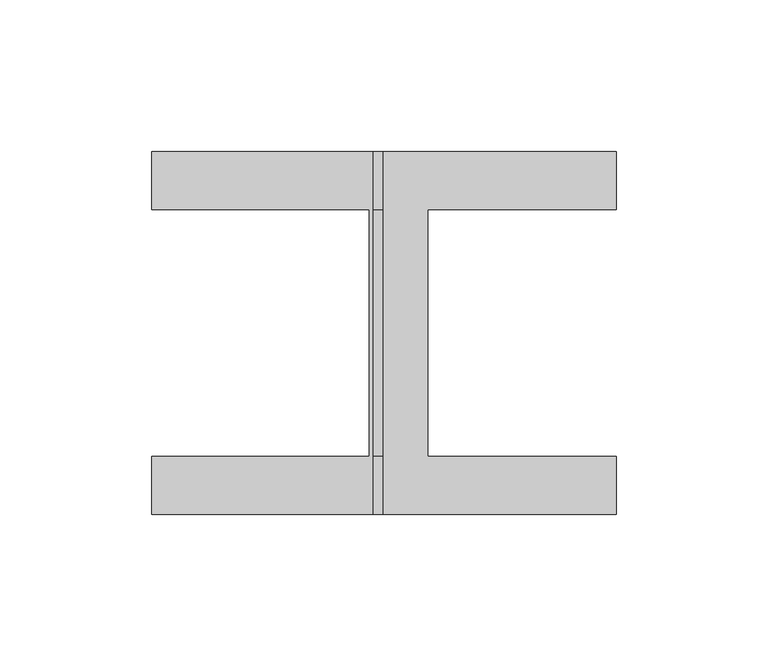
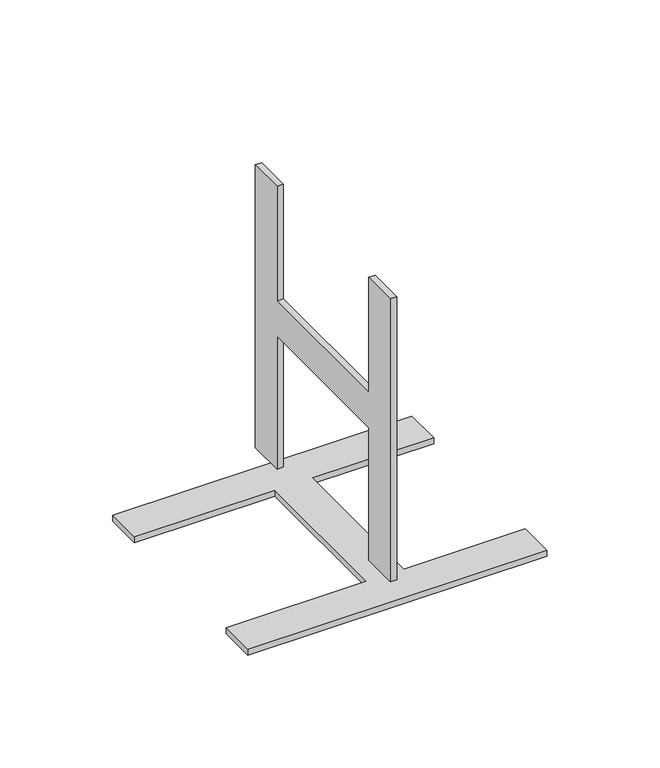
"""IFC4 building model written with IfcOpenShell, lengths in millimetres: proxy geometry, Grid Number2_FedEx : Grid Number2_FedEx."""

import ifcopenshell
import ifcopenshell.guid

model = None  # the IFC model being written
_history = None  # IfcOwnerHistory: only IFC2X3 demands one
_inside = {}  # id of a spatial element -> (the spatial element, [elements in it])
_under = {}  # id of a project, library or spatial element -> (it, [spatial elements below it])
_declared = {}  # id of a project -> (the project, [libraries it declares])
_typed = {}  # id of a type object -> (the type object, [elements of that type])
_made_of = {}  # id of a material, layer set ... -> (it, [elements and type objects made of it])


def new_model(schema):
    """Start an empty IFC model of exactly this schema.

    Asked for "IFC4X3", IfcOpenShell would pick the latest addendum, in which some entities
    have other attributes; the version numbers below select the first issue.
    IFC2X3 requires an IfcOwnerHistory on every rooted entity: one is made here for all.
    """
    global model, _history
    if schema == "IFC4X3":
        model = ifcopenshell.file(schema_version=(4, 3, 0, 0))
    else:
        model = ifcopenshell.file(schema=schema)
    _inside.clear()
    _under.clear()
    _declared.clear()
    _typed.clear()
    _made_of.clear()
    _history = None
    if model.schema == "IFC2X3":
        org = make("IfcOrganization", Name="unknown")
        user = make(
            "IfcPersonAndOrganization",
            ThePerson=make("IfcPerson", FamilyName="unknown"),
            TheOrganization=org,
        )
        app = make(
            "IfcApplication",
            ApplicationDeveloper=org,
            Version="unknown",
            ApplicationFullName="unknown",
            ApplicationIdentifier="unknown",
        )
        _history = make(
            "IfcOwnerHistory",
            OwningUser=user,
            OwningApplication=app,
            ChangeAction="ADDED",
            CreationDate=0,
        )
    return model


def make(cls, **values):
    """One entity of the class cls with the attributes given. An attribute that is None is left unset."""
    return model.create_entity(
        cls, **{name: value for name, value in values.items() if value is not None}
    )


def rooted(cls, **values):
    """An entity with a GlobalId (a new one), such as an element, a storey or a relation."""
    return make(cls, GlobalId=ifcopenshell.guid.new(), OwnerHistory=_history, **values)


def si_unit(unit_type, name, prefix=None):
    """IfcSIUnit, for example si_unit("LENGTHUNIT", "METRE", prefix="MILLI")."""
    return make("IfcSIUnit", UnitType=unit_type, Prefix=prefix, Name=name)


def assignment(units):
    """IfcUnitAssignment: the units of a project."""
    return None if units is None else make("IfcUnitAssignment", Units=units)


def point(xyz):
    """IfcCartesianPoint."""
    return None if xyz is None else make("IfcCartesianPoint", Coordinates=xyz)


def direction(xyz):
    """IfcDirection."""
    return None if xyz is None else make("IfcDirection", DirectionRatios=xyz)


def frame(location, z_axis=None, x_axis=None):
    """IfcAxis2Placement3D, a coordinate frame: its origin and axes. An axis left out is left unset."""
    return make(
        "IfcAxis2Placement3D",
        Location=point(location),
        Axis=direction(z_axis),
        RefDirection=direction(x_axis),
    )


def origin():
    """The frame at (0, 0, 0) with its axes left unset."""
    return frame((0.0, 0.0, 0.0))


def origin_with_axes():
    """The frame at (0, 0, 0) with the z axis (0, 0, 1) and the x axis (1, 0, 0) written out."""
    return frame((0.0, 0.0, 0.0), z_axis=(0.0, 0.0, 1.0), x_axis=(1.0, 0.0, 0.0))


def place(relative_to, where):
    """IfcLocalPlacement: puts the frame where relative to a parent placement (None: the world)."""
    return make(
        "IfcLocalPlacement", PlacementRelTo=relative_to, RelativePlacement=where
    )


def context(
    kind, dimensions, precision=None, world=None, true_north=None, identifier=None
):
    """IfcGeometricRepresentationContext, for example the 3D "Model" context."""
    return make(
        "IfcGeometricRepresentationContext",
        ContextIdentifier=identifier,
        ContextType=kind,
        CoordinateSpaceDimension=dimensions,
        Precision=precision,
        WorldCoordinateSystem=world,
        TrueNorth=true_north,
    )


def project(units=None, contexts=None):
    """IfcProject with its units and contexts."""
    return rooted(
        "IfcProject",
        Name="project",
        RepresentationContexts=contexts,
        UnitsInContext=assignment(units),
    )


def spatial(cls, under=None, at=None, **own):
    """A site, building, storey or space (cls), placed at a placement, below another one or the project."""
    s = rooted(cls, ObjectPlacement=at, **own)
    if under is not None:
        _under.setdefault(under.id(), (under, []))[1].append(s)
    return s


def polyline(points):
    """IfcPolyline through the points."""
    return make("IfcPolyline", Points=[point(p) for p in points])


def outline(outer, holes=None, kind="AREA"):
    """IfcArbitraryClosedProfileDef: a profile drawn as a closed curve; with holes, ...WithVoids."""
    if holes is None:
        return make("IfcArbitraryClosedProfileDef", ProfileType=kind, OuterCurve=outer)
    return make(
        "IfcArbitraryProfileDefWithVoids",
        ProfileType=kind,
        OuterCurve=outer,
        InnerCurves=holes,
    )


def extrude(swept, where, along, depth):
    """IfcExtrudedAreaSolid: the profile swept, set in the frame where, extruded along a direction by depth."""
    return make(
        "IfcExtrudedAreaSolid",
        SweptArea=swept,
        Position=where,
        ExtrudedDirection=direction(along),
        Depth=depth,
    )


def shape(context_of_items, identifier, shape_type, items):
    """IfcShapeRepresentation: the items that make up one representation, for example the "Body"."""
    return make(
        "IfcShapeRepresentation",
        ContextOfItems=context_of_items,
        RepresentationIdentifier=identifier,
        RepresentationType=shape_type,
        Items=items,
    )


def source(mapping_origin, context_of_items, identifier, shape_type, items):
    """IfcRepresentationMap: a shape defined once, which mapped items show again and again."""
    return make(
        "IfcRepresentationMap",
        MappingOrigin=mapping_origin,
        MappedRepresentation=shape(context_of_items, identifier, shape_type, items),
    )


def transform(
    local_origin,
    x_axis=None,
    y_axis=None,
    z_axis=None,
    scale=None,
    scale2=None,
    scale3=None,
    uniform=True,
):
    """IfcCartesianTransformationOperator3D, or its non-uniform kind. x_axis, y_axis, z_axis: its Axis1, 2, 3."""
    if uniform:
        return make(
            "IfcCartesianTransformationOperator3D",
            Axis1=direction(x_axis),
            Axis2=direction(y_axis),
            LocalOrigin=point(local_origin),
            Scale=scale,
            Axis3=direction(z_axis),
        )
    return make(
        "IfcCartesianTransformationOperator3DnonUniform",
        Axis1=direction(x_axis),
        Axis2=direction(y_axis),
        LocalOrigin=point(local_origin),
        Scale=scale,
        Axis3=direction(z_axis),
        Scale2=scale2,
        Scale3=scale3,
    )


def mapped(mapping_source, mapping_target):
    """IfcMappedItem: shows the shape of a source again, moved by a transform."""
    return make(
        "IfcMappedItem", MappingSource=mapping_source, MappingTarget=mapping_target
    )


def made_of(thing, what):
    """Note that an element or type object is made of a material, layer set ...; save() writes the relation."""
    if what is not None:
        _made_of.setdefault(what.id(), (what, []))[1].append(thing)
    return thing


def element(
    cls,
    number,
    at=None,
    inside=None,
    cuts=None,
    type_object=None,
    material=None,
    context=None,
    identifier="Body",
    shape_type=None,
    held_by="IfcProductDefinitionShape",
    body=None,
    shapes=None,
    **own,
):
    """One element of the class cls, such as IfcWall. Its Tag is "e" and its number.

    at: its placement. inside: the storey or other place that contains it. cuts: it is an
    opening in that element (IfcRelVoidsElement). A single representation is given by context,
    identifier, shape_type and body (its items); several are given by shapes. held_by: the class
    of the entity that holds the representations. save() writes the other relations.
    """
    e = rooted(cls, Tag="e%d" % number, ObjectPlacement=at, **own)
    if body is not None:
        shapes = [shape(context, identifier, shape_type, body)]
    if shapes is not None:
        e.Representation = make(held_by, Representations=shapes)
    if inside is not None:
        _inside.setdefault(inside.id(), (inside, []))[1].append(e)
    if cuts is not None:
        rooted(
            "IfcRelVoidsElement", RelatingBuildingElement=cuts, RelatedOpeningElement=e
        )
    if type_object is not None:
        _typed.setdefault(type_object.id(), (type_object, []))[1].append(e)
    return made_of(e, material)


def aggregate(whole, parts):
    """IfcRelAggregates: a whole, such as a stair, and the parts it consists of."""
    return rooted("IfcRelAggregates", RelatingObject=whole, RelatedObjects=parts)


def save(model, path):
    """Write the relations noted so far, then the file.

    IfcRelAggregates (storeys below a building ...), IfcRelContainedInSpatialStructure (elements
    in a storey), IfcRelDefinesByType, IfcRelAssociatesMaterial and IfcRelDeclares: one each for
    every whole, place, type object, material and project.
    """
    for whole, parts in _under.values():
        aggregate(whole, parts)
    for where, things in _inside.values():
        rooted(
            "IfcRelContainedInSpatialStructure",
            RelatedElements=things,
            RelatingStructure=where,
        )
    for kind, things in _typed.values():
        rooted("IfcRelDefinesByType", RelatedObjects=things, RelatingType=kind)
    for what, things in _made_of.values():
        rooted("IfcRelAssociatesMaterial", RelatedObjects=things, RelatingMaterial=what)
    for by, libraries in _declared.values():
        rooted("IfcRelDeclares", RelatingContext=by, RelatedDefinitions=libraries)
    model.write(path)


def entourage_b8f02744(model_context):
    return source(origin(), model_context, "Body", "SweptSolid", [
        extrude(outline(polyline([(-184.2739267, 282.3235737), (-31.1785101, 282.3235737), (-31.1785101, 263.1866466), (-93.3735231, 263.1866466), (-93.3735231, 181.8547065), (-31.1785101, 181.8547065), (-31.1785101, 162.7177794), (-184.2739267, 162.7177794), (-184.2739267, 181.8547065), (-112.5104502, 181.8547065), (-112.5104502, 263.1866466), (-184.2739267, 263.1866466), (-184.2739267, 282.3235737)])), origin_with_axes(), (0.0, 0.0, 1.0), 3.175),
        extrude(outline(polyline([(282.3235737, 14.2382753), (263.1866466, 14.2382753), (263.1866466, 86.0017519), (181.8547065, 86.0017519), (181.8547065, 14.2382753), (162.7177794, 14.2382753), (162.7177794, 167.333692), (181.8547065, 167.333692), (181.8547065, 105.138679), (263.1866466, 105.138679), (263.1866466, 167.333692), (282.3235737, 167.333692), (282.3235737, 14.2382753)])), frame((-111.2489267, 0.0, 0.0), z_axis=(1.0, 0.0, 0.0), x_axis=(0.0, 1.0, 0.0)), (0.0, 0.0, 1.0), 3.175),
    ])


if __name__ == "__main__":
    model = new_model("IFC4")
    model_context = context("Model", 3, world=origin())
    ifc_project = project(units=[si_unit("LENGTHUNIT", "METRE", prefix="MILLI")], contexts=[model_context])
    site = spatial("IfcSite", under=ifc_project)
    building = spatial("IfcBuilding", under=site)
    placement = place(None, origin())
    entourage_shape = entourage_b8f02744(model_context)
    element("IfcBuildingElementProxy", 1, Name="Grid Number2_FedEx : Grid Number2_FedEx", ObjectType="Grid Number2_FedEx : Grid Number2_FedEx", at=placement, inside=building, context=model_context, shape_type="MappedRepresentation", body=[
        mapped(entourage_shape, transform((0.0, 0.0, 0.0), x_axis=(1.0, 0.0, 0.0), y_axis=(0.0, 1.0, 0.0), z_axis=(0.0, 0.0, 1.0))),
    ])
    save(model, "model.ifc")

# Revit data of these elements
# Type "Grid Number2_FedEx : Grid Number2_FedEx"
#   Grid [instance default] = "S"
#   Label Width [instance default] = 1' - 0"
#   Half Box Width2 [instance default] = 0' - 6.13846"
#   Half Box Width [instance default] = 0' - 6"
#   Robust [instance default] = yes
#   Height = 0
#   Assembly Code = ""
# Element 1 (IfcBuildingElementProxy, "Grid Number2_FedEx : Grid Number2_FedEx")
#   Grid = "H"
#   Robust = no
#   Materials on its faces: "Letter"
# Materials
#   "Letter": class "Unassigned", colour RGB 178 187 30, transparency 0, Comments = "Rendering appearance not upgraded "
